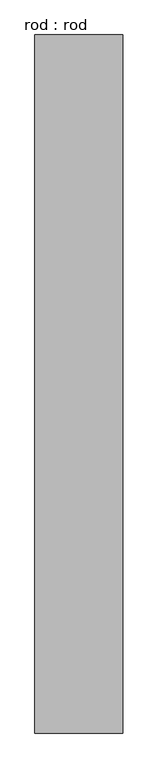
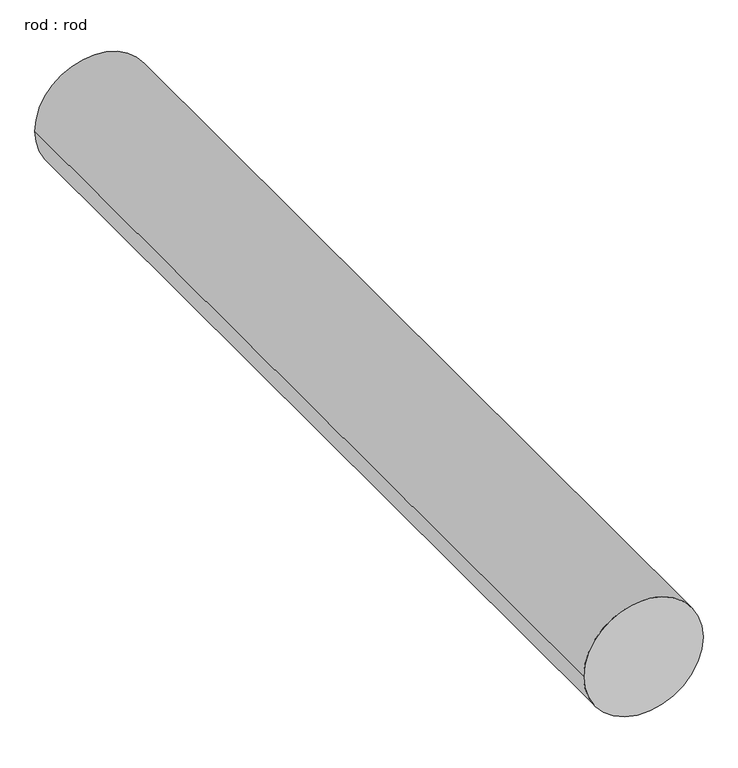
"""IFC4 building model written with IfcOpenShell, lengths in millimetres: proxy geometry, rod : rod."""

from ifc_helpers import new_model, si_unit, point, frame, frame_2d, origin, place, context, project, spatial, circle_curve, trimmed, segment, composite_curve, outline, extrude, source, transform, mapped, element, save


def rod_rod_c5f87591(model_context):
    return source(origin(), model_context, "Body", "SweptSolid", [
        extrude(outline(composite_curve([segment(trimmed(circle_curve(frame_2d((0.0108462, 0.0)), 200.0), [point((0.0108462, 200.0))], [point((0.0108462, -200.0))], False, "CARTESIAN"), True, "CONTINUOUS"), segment(trimmed(circle_curve(frame_2d((0.0108462, 0.0)), 200.0), [point((0.0108462, -200.0))], [point((0.0108462, 200.0))], False, "CARTESIAN"), True, "CONTINUOUS")], self_intersect=False)), frame((0.0, 2501.6571868, 0.0), z_axis=(0.0, 1.0, 0.0), x_axis=(0.0, 0.0, 1.0)), (0.0, 0.0, 1.0), 3182.1428571),
    ])


if __name__ == "__main__":
    model = new_model("IFC4")
    model_context = context("Model", 3, world=origin())
    ifc_project = project(units=[si_unit("LENGTHUNIT", "METRE", prefix="MILLI")], contexts=[model_context])
    site = spatial("IfcSite", under=ifc_project)
    building = spatial("IfcBuilding", under=site)
    placement = place(None, origin())
    rod_rod_shape = rod_rod_c5f87591(model_context)
    element("IfcBuildingElementProxy", 1, Name="rod : rod", ObjectType="rod : rod", at=placement, inside=building, context=model_context, shape_type="MappedRepresentation", body=[
        mapped(rod_rod_shape, transform((0.0, 0.0, 0.0), x_axis=(1.0, 0.0, 0.0), y_axis=(0.0, 1.0, 0.0), z_axis=(0.0, 0.0, 1.0))),
    ])
    save(model, "model.ifc")

# Revit data of these elements
# Type "rod : rod"
#   Default Elevation = 0
